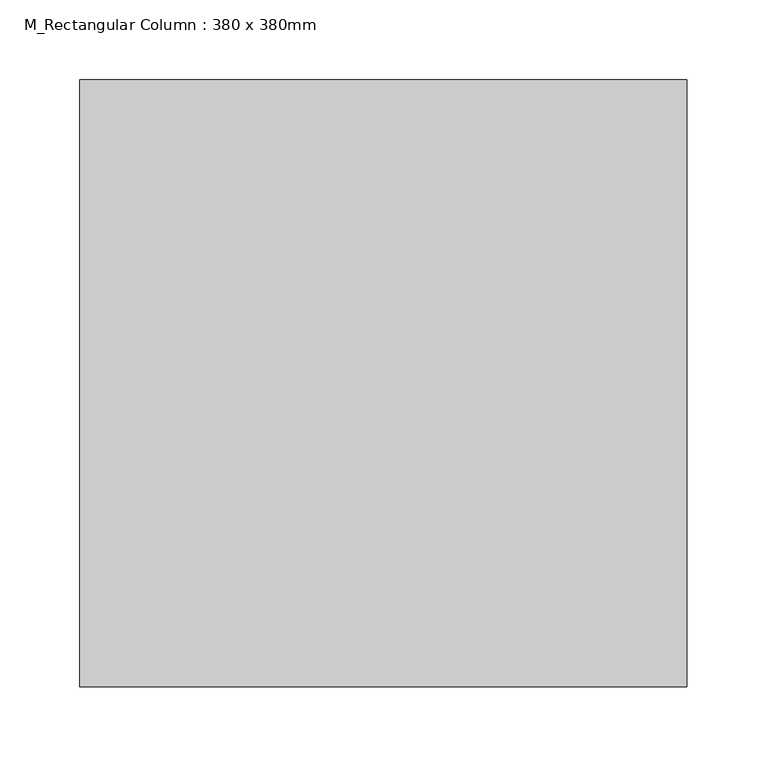
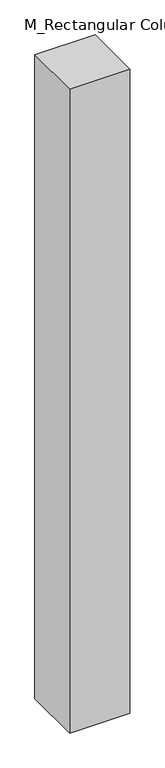
"""IFC4 building model written with IfcOpenShell, lengths in millimetres: column geometry, M_Rectangular Column : 380 x 380mm."""

import ifcopenshell
import ifcopenshell.guid

model = None  # the IFC model being written
_history = None  # IfcOwnerHistory: only IFC2X3 demands one
_inside = {}  # id of a spatial element -> (the spatial element, [elements in it])
_under = {}  # id of a project, library or spatial element -> (it, [spatial elements below it])
_declared = {}  # id of a project -> (the project, [libraries it declares])
_typed = {}  # id of a type object -> (the type object, [elements of that type])
_made_of = {}  # id of a material, layer set ... -> (it, [elements and type objects made of it])


def new_model(schema):
    """Start an empty IFC model of exactly this schema.

    Asked for "IFC4X3", IfcOpenShell would pick the latest addendum, in which some entities
    have other attributes; the version numbers below select the first issue.
    IFC2X3 requires an IfcOwnerHistory on every rooted entity: one is made here for all.
    """
    global model, _history
    if schema == "IFC4X3":
        model = ifcopenshell.file(schema_version=(4, 3, 0, 0))
    else:
        model = ifcopenshell.file(schema=schema)
    _inside.clear()
    _under.clear()
    _declared.clear()
    _typed.clear()
    _made_of.clear()
    _history = None
    if model.schema == "IFC2X3":
        org = make("IfcOrganization", Name="unknown")
        user = make(
            "IfcPersonAndOrganization",
            ThePerson=make("IfcPerson", FamilyName="unknown"),
            TheOrganization=org,
        )
        app = make(
            "IfcApplication",
            ApplicationDeveloper=org,
            Version="unknown",
            ApplicationFullName="unknown",
            ApplicationIdentifier="unknown",
        )
        _history = make(
            "IfcOwnerHistory",
            OwningUser=user,
            OwningApplication=app,
            ChangeAction="ADDED",
            CreationDate=0,
        )
    return model


def make(cls, **values):
    """One entity of the class cls with the attributes given. An attribute that is None is left unset."""
    return model.create_entity(
        cls, **{name: value for name, value in values.items() if value is not None}
    )


def rooted(cls, **values):
    """An entity with a GlobalId (a new one), such as an element, a storey or a relation."""
    return make(cls, GlobalId=ifcopenshell.guid.new(), OwnerHistory=_history, **values)


def si_unit(unit_type, name, prefix=None):
    """IfcSIUnit, for example si_unit("LENGTHUNIT", "METRE", prefix="MILLI")."""
    return make("IfcSIUnit", UnitType=unit_type, Prefix=prefix, Name=name)


def assignment(units):
    """IfcUnitAssignment: the units of a project."""
    return None if units is None else make("IfcUnitAssignment", Units=units)


def point(xyz):
    """IfcCartesianPoint."""
    return None if xyz is None else make("IfcCartesianPoint", Coordinates=xyz)


def direction(xyz):
    """IfcDirection."""
    return None if xyz is None else make("IfcDirection", DirectionRatios=xyz)


def frame(location, z_axis=None, x_axis=None):
    """IfcAxis2Placement3D, a coordinate frame: its origin and axes. An axis left out is left unset."""
    return make(
        "IfcAxis2Placement3D",
        Location=point(location),
        Axis=direction(z_axis),
        RefDirection=direction(x_axis),
    )


def origin():
    """The frame at (0, 0, 0) with its axes left unset."""
    return frame((0.0, 0.0, 0.0))


def origin_with_axes():
    """The frame at (0, 0, 0) with the z axis (0, 0, 1) and the x axis (1, 0, 0) written out."""
    return frame((0.0, 0.0, 0.0), z_axis=(0.0, 0.0, 1.0), x_axis=(1.0, 0.0, 0.0))


def place(relative_to, where):
    """IfcLocalPlacement: puts the frame where relative to a parent placement (None: the world)."""
    return make(
        "IfcLocalPlacement", PlacementRelTo=relative_to, RelativePlacement=where
    )


def context(
    kind, dimensions, precision=None, world=None, true_north=None, identifier=None
):
    """IfcGeometricRepresentationContext, for example the 3D "Model" context."""
    return make(
        "IfcGeometricRepresentationContext",
        ContextIdentifier=identifier,
        ContextType=kind,
        CoordinateSpaceDimension=dimensions,
        Precision=precision,
        WorldCoordinateSystem=world,
        TrueNorth=true_north,
    )


def project(units=None, contexts=None):
    """IfcProject with its units and contexts."""
    return rooted(
        "IfcProject",
        Name="project",
        RepresentationContexts=contexts,
        UnitsInContext=assignment(units),
    )


def spatial(cls, under=None, at=None, **own):
    """A site, building, storey or space (cls), placed at a placement, below another one or the project."""
    s = rooted(cls, ObjectPlacement=at, **own)
    if under is not None:
        _under.setdefault(under.id(), (under, []))[1].append(s)
    return s


def polyline(points):
    """IfcPolyline through the points."""
    return make("IfcPolyline", Points=[point(p) for p in points])


def outline(outer, holes=None, kind="AREA"):
    """IfcArbitraryClosedProfileDef: a profile drawn as a closed curve; with holes, ...WithVoids."""
    if holes is None:
        return make("IfcArbitraryClosedProfileDef", ProfileType=kind, OuterCurve=outer)
    return make(
        "IfcArbitraryProfileDefWithVoids",
        ProfileType=kind,
        OuterCurve=outer,
        InnerCurves=holes,
    )


def extrude(swept, where, along, depth):
    """IfcExtrudedAreaSolid: the profile swept, set in the frame where, extruded along a direction by depth."""
    return make(
        "IfcExtrudedAreaSolid",
        SweptArea=swept,
        Position=where,
        ExtrudedDirection=direction(along),
        Depth=depth,
    )


def shape(context_of_items, identifier, shape_type, items):
    """IfcShapeRepresentation: the items that make up one representation, for example the "Body"."""
    return make(
        "IfcShapeRepresentation",
        ContextOfItems=context_of_items,
        RepresentationIdentifier=identifier,
        RepresentationType=shape_type,
        Items=items,
    )


def source(mapping_origin, context_of_items, identifier, shape_type, items):
    """IfcRepresentationMap: a shape defined once, which mapped items show again and again."""
    return make(
        "IfcRepresentationMap",
        MappingOrigin=mapping_origin,
        MappedRepresentation=shape(context_of_items, identifier, shape_type, items),
    )


def transform(
    local_origin,
    x_axis=None,
    y_axis=None,
    z_axis=None,
    scale=None,
    scale2=None,
    scale3=None,
    uniform=True,
):
    """IfcCartesianTransformationOperator3D, or its non-uniform kind. x_axis, y_axis, z_axis: its Axis1, 2, 3."""
    if uniform:
        return make(
            "IfcCartesianTransformationOperator3D",
            Axis1=direction(x_axis),
            Axis2=direction(y_axis),
            LocalOrigin=point(local_origin),
            Scale=scale,
            Axis3=direction(z_axis),
        )
    return make(
        "IfcCartesianTransformationOperator3DnonUniform",
        Axis1=direction(x_axis),
        Axis2=direction(y_axis),
        LocalOrigin=point(local_origin),
        Scale=scale,
        Axis3=direction(z_axis),
        Scale2=scale2,
        Scale3=scale3,
    )


def mapped(mapping_source, mapping_target):
    """IfcMappedItem: shows the shape of a source again, moved by a transform."""
    return make(
        "IfcMappedItem", MappingSource=mapping_source, MappingTarget=mapping_target
    )


def made_of(thing, what):
    """Note that an element or type object is made of a material, layer set ...; save() writes the relation."""
    if what is not None:
        _made_of.setdefault(what.id(), (what, []))[1].append(thing)
    return thing


def element(
    cls,
    number,
    at=None,
    inside=None,
    cuts=None,
    type_object=None,
    material=None,
    context=None,
    identifier="Body",
    shape_type=None,
    held_by="IfcProductDefinitionShape",
    body=None,
    shapes=None,
    **own,
):
    """One element of the class cls, such as IfcWall. Its Tag is "e" and its number.

    at: its placement. inside: the storey or other place that contains it. cuts: it is an
    opening in that element (IfcRelVoidsElement). A single representation is given by context,
    identifier, shape_type and body (its items); several are given by shapes. held_by: the class
    of the entity that holds the representations. save() writes the other relations.
    """
    e = rooted(cls, Tag="e%d" % number, ObjectPlacement=at, **own)
    if body is not None:
        shapes = [shape(context, identifier, shape_type, body)]
    if shapes is not None:
        e.Representation = make(held_by, Representations=shapes)
    if inside is not None:
        _inside.setdefault(inside.id(), (inside, []))[1].append(e)
    if cuts is not None:
        rooted(
            "IfcRelVoidsElement", RelatingBuildingElement=cuts, RelatedOpeningElement=e
        )
    if type_object is not None:
        _typed.setdefault(type_object.id(), (type_object, []))[1].append(e)
    return made_of(e, material)


def aggregate(whole, parts):
    """IfcRelAggregates: a whole, such as a stair, and the parts it consists of."""
    return rooted("IfcRelAggregates", RelatingObject=whole, RelatedObjects=parts)


def save(model, path):
    """Write the relations noted so far, then the file.

    IfcRelAggregates (storeys below a building ...), IfcRelContainedInSpatialStructure (elements
    in a storey), IfcRelDefinesByType, IfcRelAssociatesMaterial and IfcRelDeclares: one each for
    every whole, place, type object, material and project.
    """
    for whole, parts in _under.values():
        aggregate(whole, parts)
    for where, things in _inside.values():
        rooted(
            "IfcRelContainedInSpatialStructure",
            RelatedElements=things,
            RelatingStructure=where,
        )
    for kind, things in _typed.values():
        rooted("IfcRelDefinesByType", RelatedObjects=things, RelatingType=kind)
    for what, things in _made_of.values():
        rooted("IfcRelAssociatesMaterial", RelatedObjects=things, RelatingMaterial=what)
    for by, libraries in _declared.values():
        rooted("IfcRelDeclares", RelatingContext=by, RelatedDefinitions=libraries)
    model.write(path)


def m_rectangular_column_380_x_380mm_96b74405(model_context):
    return source(origin(), model_context, "Body", "SweptSolid", [
        extrude(outline(polyline([(190.0, 190.0), (190.0, -190.0), (-190.0, -190.0), (-190.0, 190.0), (190.0, 190.0)])), origin_with_axes(), (0.0, 0.0, 1.0), 4300.0),
    ])


if __name__ == "__main__":
    model = new_model("IFC4")
    model_context = context("Model", 3, world=origin())
    ifc_project = project(units=[si_unit("LENGTHUNIT", "METRE", prefix="MILLI")], contexts=[model_context])
    site = spatial("IfcSite", under=ifc_project)
    building = spatial("IfcBuilding", under=site)
    placement = place(None, origin())
    m_rectangular_column_380_x_380mm_shape = m_rectangular_column_380_x_380mm_96b74405(model_context)
    element("IfcColumn", 1, ObjectType="M_Rectangular Column : 380 x 380mm", at=placement, inside=building, context=model_context, shape_type="MappedRepresentation", body=[
        mapped(m_rectangular_column_380_x_380mm_shape, transform((0.0, 0.0, 0.0), x_axis=(1.0, 0.0, 0.0), y_axis=(0.0, 1.0, 0.0), z_axis=(0.0, 0.0, 1.0))),
    ])
    save(model, "model.ifc")

# Revit data of these elements
# Type "M_Rectangular Column : 380 x 380mm"
#   Depth = 38 cm
#   Offset Base = 0 cm
#   Offset Top = 0 cm
#   Width = 38 cm
#   Material = none
